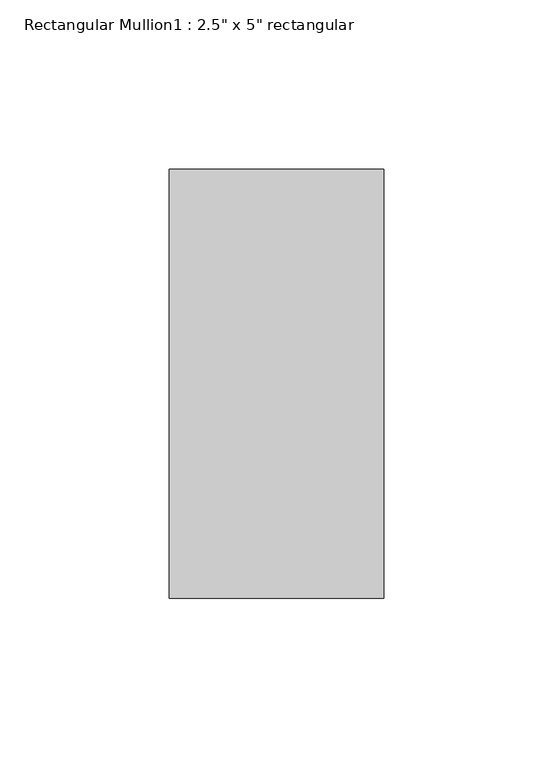
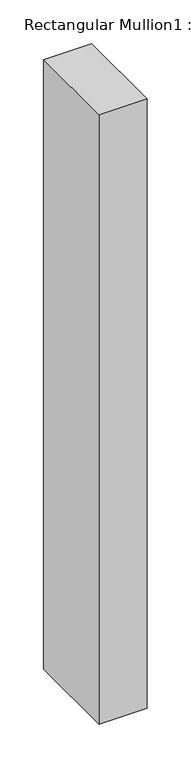
"""IFC4 building model written with IfcOpenShell, lengths in millimetres: member geometry."""

from ifc_helpers import new_model, si_unit, frame, origin, place, context, project, spatial, polyline, outline, extrude, source, transform, mapped, element, save


def member_d2e7e466(model_context):
    return source(origin(), model_context, "Body", "SweptSolid", [
        extrude(outline(polyline([(0.0, 63.5), (0.0, -63.5), (-63.5, -63.5), (-63.5, 63.5), (0.0, 63.5)])), frame((0.0, 0.0, -850.9), z_axis=(0.0, 0.0, 1.0), x_axis=(1.0, 0.0, 0.0)), (0.0, 0.0, 1.0), 850.9),
    ])


if __name__ == "__main__":
    model = new_model("IFC4")
    model_context = context("Model", 3, world=origin())
    ifc_project = project(units=[si_unit("LENGTHUNIT", "METRE", prefix="MILLI")], contexts=[model_context])
    site = spatial("IfcSite", under=ifc_project)
    building = spatial("IfcBuilding", under=site)
    placement = place(None, origin())
    member_shape = member_d2e7e466(model_context)
    element("IfcMember", 1, ObjectType="Rectangular Mullion1 : 2.5\" x 5\" rectangular", at=placement, inside=building, context=model_context, shape_type="MappedRepresentation", body=[
        mapped(member_shape, transform((0.0, 0.0, 0.0), x_axis=(1.0, 0.0, 0.0), y_axis=(0.0, 1.0, 0.0), z_axis=(0.0, 0.0, 1.0))),
    ])
    save(model, "model.ifc")

# Revit data of these elements
# Type "Rectangular Mullion1 : 2.5\" x 5\" rectangular"
#   built-in parameter 1007304 = 0.416667 (stored number, unit not read)
#   built-in parameter 1007301 = 0.104167 (stored number, unit not read)
#   built-in parameter 1007300 = 0.104167 (stored number, unit not read)
# Element 1 (IfcMember, "Rectangular Mullion1 : 2.5\" x 5\" rectangular")
#   Materials on its faces: "support-frame"
# Materials
#   "support-frame": class "Unassigned", colour RGB 233 233 233, transparency 0, Cost = 0
